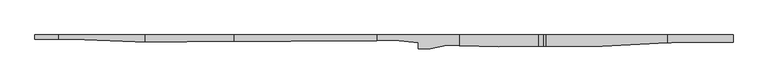
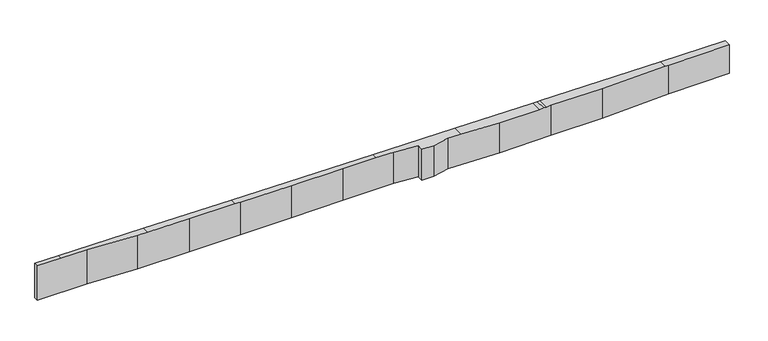
"""IFC4 building model written with IfcOpenShell, lengths in millimetres: proxy geometry, Flowable Fill : Flowable Fill."""

import ifcopenshell
import ifcopenshell.guid

model = None  # the IFC model being written
_history = None  # IfcOwnerHistory: only IFC2X3 demands one
_inside = {}  # id of a spatial element -> (the spatial element, [elements in it])
_under = {}  # id of a project, library or spatial element -> (it, [spatial elements below it])
_declared = {}  # id of a project -> (the project, [libraries it declares])
_typed = {}  # id of a type object -> (the type object, [elements of that type])
_made_of = {}  # id of a material, layer set ... -> (it, [elements and type objects made of it])


def new_model(schema):
    """Start an empty IFC model of exactly this schema.

    Asked for "IFC4X3", IfcOpenShell would pick the latest addendum, in which some entities
    have other attributes; the version numbers below select the first issue.
    IFC2X3 requires an IfcOwnerHistory on every rooted entity: one is made here for all.
    """
    global model, _history
    if schema == "IFC4X3":
        model = ifcopenshell.file(schema_version=(4, 3, 0, 0))
    else:
        model = ifcopenshell.file(schema=schema)
    _inside.clear()
    _under.clear()
    _declared.clear()
    _typed.clear()
    _made_of.clear()
    _history = None
    if model.schema == "IFC2X3":
        org = make("IfcOrganization", Name="unknown")
        user = make(
            "IfcPersonAndOrganization",
            ThePerson=make("IfcPerson", FamilyName="unknown"),
            TheOrganization=org,
        )
        app = make(
            "IfcApplication",
            ApplicationDeveloper=org,
            Version="unknown",
            ApplicationFullName="unknown",
            ApplicationIdentifier="unknown",
        )
        _history = make(
            "IfcOwnerHistory",
            OwningUser=user,
            OwningApplication=app,
            ChangeAction="ADDED",
            CreationDate=0,
        )
    return model


def make(cls, **values):
    """One entity of the class cls with the attributes given. An attribute that is None is left unset."""
    return model.create_entity(
        cls, **{name: value for name, value in values.items() if value is not None}
    )


def rooted(cls, **values):
    """An entity with a GlobalId (a new one), such as an element, a storey or a relation."""
    return make(cls, GlobalId=ifcopenshell.guid.new(), OwnerHistory=_history, **values)


def si_unit(unit_type, name, prefix=None):
    """IfcSIUnit, for example si_unit("LENGTHUNIT", "METRE", prefix="MILLI")."""
    return make("IfcSIUnit", UnitType=unit_type, Prefix=prefix, Name=name)


def assignment(units):
    """IfcUnitAssignment: the units of a project."""
    return None if units is None else make("IfcUnitAssignment", Units=units)


def point(xyz):
    """IfcCartesianPoint."""
    return None if xyz is None else make("IfcCartesianPoint", Coordinates=xyz)


def direction(xyz):
    """IfcDirection."""
    return None if xyz is None else make("IfcDirection", DirectionRatios=xyz)


def frame(location, z_axis=None, x_axis=None):
    """IfcAxis2Placement3D, a coordinate frame: its origin and axes. An axis left out is left unset."""
    return make(
        "IfcAxis2Placement3D",
        Location=point(location),
        Axis=direction(z_axis),
        RefDirection=direction(x_axis),
    )


def origin():
    """The frame at (0, 0, 0) with its axes left unset."""
    return frame((0.0, 0.0, 0.0))


def place(relative_to, where):
    """IfcLocalPlacement: puts the frame where relative to a parent placement (None: the world)."""
    return make(
        "IfcLocalPlacement", PlacementRelTo=relative_to, RelativePlacement=where
    )


def context(
    kind, dimensions, precision=None, world=None, true_north=None, identifier=None
):
    """IfcGeometricRepresentationContext, for example the 3D "Model" context."""
    return make(
        "IfcGeometricRepresentationContext",
        ContextIdentifier=identifier,
        ContextType=kind,
        CoordinateSpaceDimension=dimensions,
        Precision=precision,
        WorldCoordinateSystem=world,
        TrueNorth=true_north,
    )


def project(units=None, contexts=None):
    """IfcProject with its units and contexts."""
    return rooted(
        "IfcProject",
        Name="project",
        RepresentationContexts=contexts,
        UnitsInContext=assignment(units),
    )


def spatial(cls, under=None, at=None, **own):
    """A site, building, storey or space (cls), placed at a placement, below another one or the project."""
    s = rooted(cls, ObjectPlacement=at, **own)
    if under is not None:
        _under.setdefault(under.id(), (under, []))[1].append(s)
    return s


def faces_of(points, faces, orient=None, outer=None):
    """IfcFace entities. A face is a list of loops; a loop is a list of indices into points, from 0.

    orient and outer hold one flag for each loop. By default every Orientation is true, the
    first loop of a face is its IfcFaceOuterBound and the others are IfcFaceBound.
    """
    made = []
    for i, loops in enumerate(faces):
        bounds = []
        for j, loop in enumerate(loops):
            is_outer = j == 0 if outer is None else outer[i][j]
            bounds.append(
                make(
                    "IfcFaceOuterBound" if is_outer else "IfcFaceBound",
                    Bound=make("IfcPolyLoop", Polygon=[points[k] for k in loop]),
                    Orientation=True if orient is None else orient[i][j],
                )
            )
        made.append(make("IfcFace", Bounds=bounds))
    return made


def faceted_brep(points, faces, orient=None, outer=None, voids=None):
    """IfcFacetedBrep: a solid bounded by flat faces; with voids (closed shells), ...WithVoids."""
    shared = [point(p) for p in points]
    hull = make("IfcClosedShell", CfsFaces=faces_of(shared, faces, orient, outer))
    if voids is None:
        return make("IfcFacetedBrep", Outer=hull)
    return make(
        "IfcFacetedBrepWithVoids",
        Outer=hull,
        Voids=[
            make(cls, CfsFaces=faces_of(shared, fs, o, b)) for cls, fs, o, b in voids
        ],
    )


def shape(context_of_items, identifier, shape_type, items):
    """IfcShapeRepresentation: the items that make up one representation, for example the "Body"."""
    return make(
        "IfcShapeRepresentation",
        ContextOfItems=context_of_items,
        RepresentationIdentifier=identifier,
        RepresentationType=shape_type,
        Items=items,
    )


def source(mapping_origin, context_of_items, identifier, shape_type, items):
    """IfcRepresentationMap: a shape defined once, which mapped items show again and again."""
    return make(
        "IfcRepresentationMap",
        MappingOrigin=mapping_origin,
        MappedRepresentation=shape(context_of_items, identifier, shape_type, items),
    )


def transform(
    local_origin,
    x_axis=None,
    y_axis=None,
    z_axis=None,
    scale=None,
    scale2=None,
    scale3=None,
    uniform=True,
):
    """IfcCartesianTransformationOperator3D, or its non-uniform kind. x_axis, y_axis, z_axis: its Axis1, 2, 3."""
    if uniform:
        return make(
            "IfcCartesianTransformationOperator3D",
            Axis1=direction(x_axis),
            Axis2=direction(y_axis),
            LocalOrigin=point(local_origin),
            Scale=scale,
            Axis3=direction(z_axis),
        )
    return make(
        "IfcCartesianTransformationOperator3DnonUniform",
        Axis1=direction(x_axis),
        Axis2=direction(y_axis),
        LocalOrigin=point(local_origin),
        Scale=scale,
        Axis3=direction(z_axis),
        Scale2=scale2,
        Scale3=scale3,
    )


def mapped(mapping_source, mapping_target):
    """IfcMappedItem: shows the shape of a source again, moved by a transform."""
    return make(
        "IfcMappedItem", MappingSource=mapping_source, MappingTarget=mapping_target
    )


def made_of(thing, what):
    """Note that an element or type object is made of a material, layer set ...; save() writes the relation."""
    if what is not None:
        _made_of.setdefault(what.id(), (what, []))[1].append(thing)
    return thing


def element(
    cls,
    number,
    at=None,
    inside=None,
    cuts=None,
    type_object=None,
    material=None,
    context=None,
    identifier="Body",
    shape_type=None,
    held_by="IfcProductDefinitionShape",
    body=None,
    shapes=None,
    **own,
):
    """One element of the class cls, such as IfcWall. Its Tag is "e" and its number.

    at: its placement. inside: the storey or other place that contains it. cuts: it is an
    opening in that element (IfcRelVoidsElement). A single representation is given by context,
    identifier, shape_type and body (its items); several are given by shapes. held_by: the class
    of the entity that holds the representations. save() writes the other relations.
    """
    e = rooted(cls, Tag="e%d" % number, ObjectPlacement=at, **own)
    if body is not None:
        shapes = [shape(context, identifier, shape_type, body)]
    if shapes is not None:
        e.Representation = make(held_by, Representations=shapes)
    if inside is not None:
        _inside.setdefault(inside.id(), (inside, []))[1].append(e)
    if cuts is not None:
        rooted(
            "IfcRelVoidsElement", RelatingBuildingElement=cuts, RelatedOpeningElement=e
        )
    if type_object is not None:
        _typed.setdefault(type_object.id(), (type_object, []))[1].append(e)
    return made_of(e, material)


def aggregate(whole, parts):
    """IfcRelAggregates: a whole, such as a stair, and the parts it consists of."""
    return rooted("IfcRelAggregates", RelatingObject=whole, RelatedObjects=parts)


def save(model, path):
    """Write the relations noted so far, then the file.

    IfcRelAggregates (storeys below a building ...), IfcRelContainedInSpatialStructure (elements
    in a storey), IfcRelDefinesByType, IfcRelAssociatesMaterial and IfcRelDeclares: one each for
    every whole, place, type object, material and project.
    """
    for whole, parts in _under.values():
        aggregate(whole, parts)
    for where, things in _inside.values():
        rooted(
            "IfcRelContainedInSpatialStructure",
            RelatedElements=things,
            RelatingStructure=where,
        )
    for kind, things in _typed.values():
        rooted("IfcRelDefinesByType", RelatedObjects=things, RelatingType=kind)
    for what, things in _made_of.values():
        rooted("IfcRelAssociatesMaterial", RelatedObjects=things, RelatingMaterial=what)
    for by, libraries in _declared.values():
        rooted("IfcRelDeclares", RelatingContext=by, RelatedDefinitions=libraries)
    model.write(path)


def generic_models_da6e01de(model_context):
    return source(origin(), model_context, "Body", "Brep", [
        faceted_brep([(-76504.8, -1168.4, 8756.65), (-76504.8, -685.8, 8756.65), (0.0, -685.8, 8756.65), (0.0, -1498.6, 8756.65), (-6756.4, -1549.4, 8756.65), (-14325.6, -1905.0, 8756.65), (-20015.2, -1905.0, 8756.65), (-25704.8, -1981.2, 8756.65), (-31394.4, -1828.8, 8756.65), (-33197.8, -2224.0875, 8756.65), (-34493.2, -2224.0875, 8756.65), (-34493.2, -1538.2875, 8756.65), (-37084.0, -1295.4, 8756.65), (-42773.6, -1320.8, 8756.65), (-48463.2, -1371.6, 8756.65), (-54152.8, -1371.6, 8756.65), (-59842.4, -1447.8, 8756.65), (-65532.0, -1447.8, 8756.65), (-71018.4, -1193.8, 8756.65), (-71018.4, -1193.8, 12752.9363716), (-73924.5154607, -1180.3457618, 12775.8590028), (-76504.8, -1168.4, 12775.8590028), (-65532.0, -1447.8, 12709.661173), (-59842.4, -1447.8, 12630.8044454), (-64486.32492, -1447.8, 12701.4131786), (-54152.8, -1371.6, 12547.5273927), (-54739.2258845, -1379.4539181, 12553.2130404), (-48463.2, -1371.6, 12492.3643078), (-42773.6, -1320.8, 12437.2012228), (-37084.0, -1295.4, 12386.3772486), (-39060.1554467, -1304.2221225, 12401.197803), (-25704.8, -1981.2, 12287.5909977), (-29992.6104464, -1866.3479345, 12333.1940212), (-31394.4, -1828.8, 12343.7070091), (-20015.2, -1905.0, 12254.2742414), (-20545.0629958, -1912.0963794, 12259.7009275), (-20822.3850062, -1915.8105135, 12258.8865049), (-21332.1380629, -1922.6375633, 12241.0855359), (-14325.6, -1905.0, 12196.0031916), (-6756.4, -1549.4, 12121.4878946), (-7146.1405773, -1567.70996, 12122.4734818), (0.0, -1498.6, 12104.4021161), (0.0, -685.8, 12104.4021161), (-76504.8, -685.8, 12775.8590028), (-73924.5154607, -685.8, 12775.8590028), (-64486.32492, -685.8, 12701.4131786), (-54739.2258845, -685.8, 12553.2130404), (-39060.1554467, -685.8, 12401.197803), (-29992.6104464, -685.8, 12333.1940212), (-21332.1380629, -685.8, 12241.0855359), (-20822.3850062, -685.8, 12258.8865049), (-20545.0629958, -685.8, 12259.7009275), (-7146.1405773, -685.8, 12122.4734818), (-34493.2, -1538.2875, 12366.9470503), (-34493.2, -2224.0875, 12366.9470503), (-33197.8, -2224.0875, 12357.2319511)], [[[0, 1, 2, 3, 4, 5, 6, 7, 8, 9, 10, 11, 12, 13, 14, 15, 16, 17, 18]], [[0, 18, 19, 20, 21]], [[18, 17, 22, 19]], [[17, 16, 23, 24, 22]], [[16, 15, 25, 26, 23]], [[15, 14, 27, 25]], [[14, 13, 28, 27]], [[13, 12, 29, 30, 28]], [[8, 7, 31, 32, 33]], [[7, 6, 34, 35, 36, 37, 31]], [[6, 5, 38, 34]], [[5, 4, 39, 40, 38]], [[4, 3, 41, 39]], [[3, 2, 42, 41]], [[2, 1, 43, 44, 45, 46, 47, 48, 49, 50, 51, 52, 42]], [[1, 0, 21, 43]], [[52, 40, 39, 41, 42]], [[20, 44, 43, 21]], [[44, 20, 19, 22, 24, 45]], [[45, 24, 23, 26, 46]], [[46, 26, 25, 27, 28, 30, 47]], [[47, 30, 29, 53, 54, 55, 33, 32, 48]], [[48, 32, 31, 37, 49]], [[49, 37, 36, 50]], [[50, 36, 35, 51]], [[40, 52, 51, 35, 34, 38]], [[12, 11, 53, 29]], [[11, 10, 54, 53]], [[10, 9, 55, 54]], [[9, 8, 33, 55]]]),
    ])


if __name__ == "__main__":
    model = new_model("IFC4")
    model_context = context("Model", 3, world=origin())
    ifc_project = project(units=[si_unit("LENGTHUNIT", "METRE", prefix="MILLI")], contexts=[model_context])
    site = spatial("IfcSite", under=ifc_project)
    building = spatial("IfcBuilding", under=site)
    placement = place(None, origin())
    generic_models_shape = generic_models_da6e01de(model_context)
    element("IfcBuildingElementProxy", 1, Name="Flowable Fill : Flowable Fill", ObjectType="Flowable Fill : Flowable Fill", at=placement, inside=building, context=model_context, shape_type="MappedRepresentation", body=[
        mapped(generic_models_shape, transform((0.0, 0.0, 0.0), x_axis=(1.0, 0.0, 0.0), y_axis=(0.0, 1.0, 0.0), z_axis=(0.0, 0.0, 1.0))),
    ])
    save(model, "model.ifc")

# Revit data of these elements
# Element 1 (IfcBuildingElementProxy, "Flowable Fill : Flowable Fill")
#   Materials on its faces: "Site - Flowable Fill"
# Materials
#   "Site - Flowable Fill": class "Generic", colour RGB 255 0 128, transparency 0, Cost = 0
